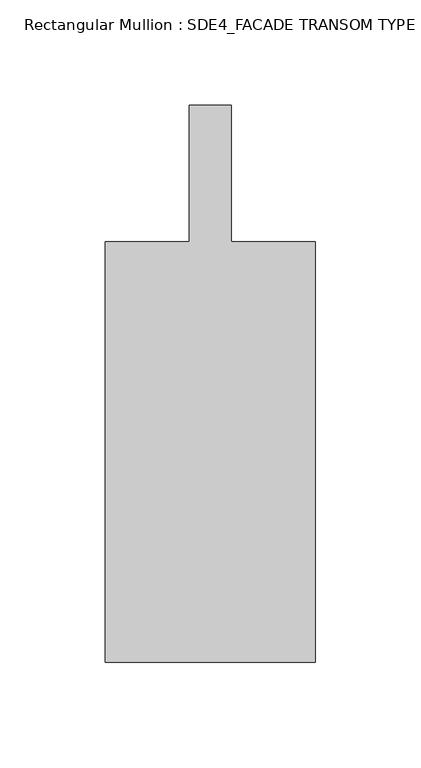
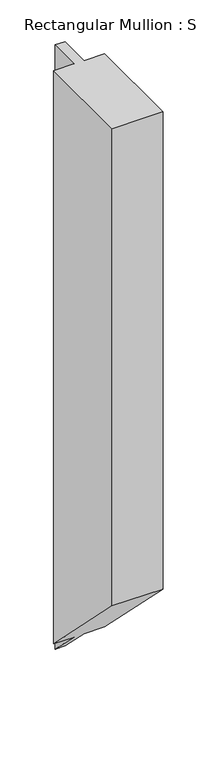
"""IFC4 building model written with IfcOpenShell, lengths in millimetres: member geometry, Rectangular Mullion : SDE4_FACADE TRANSOM TYPE 2."""

from ifc_helpers import new_model, si_unit, origin, place, context, project, spatial, faceted_brep, source, transform, mapped, element, save


def rectangular_mullion_sde4_facade_transom_type_2_1d46e8af(model_context):
    return source(origin(), model_context, "Body", "Brep", [
        faceted_brep([(50.0, -132.5, 0.0), (50.0, 67.5, 0.0), (10.0, 67.5, 0.0), (10.0, 132.5, 0.0), (-10.0, 132.5, 0.0), (-10.0, 67.5, 0.0), (-50.0, 67.5, 0.0), (-50.0, -132.5, 0.0), (50.0, -132.5, -995.0000001), (50.0, 67.5, -1195.0000001), (10.0, 67.5, -1195.0000001), (10.0, 132.5, -1260.0000001), (-10.0, 132.5, -1260.0000001), (-10.0, 67.5, -1195.0000001), (-50.0, 67.5, -1195.0000001), (-50.0, -132.5, -995.0000001)], [[[0, 1, 2, 3, 4, 5, 6, 7]], [[1, 0, 8, 9]], [[2, 1, 9, 10]], [[3, 2, 10, 11]], [[4, 3, 11, 12]], [[5, 4, 12, 13]], [[6, 5, 13, 14]], [[7, 6, 14, 15]], [[0, 7, 15, 8]], [[8, 15, 14, 13, 12, 11, 10, 9]]]),
    ])


if __name__ == "__main__":
    model = new_model("IFC4")
    model_context = context("Model", 3, world=origin())
    ifc_project = project(units=[si_unit("LENGTHUNIT", "METRE", prefix="MILLI")], contexts=[model_context])
    site = spatial("IfcSite", under=ifc_project)
    building = spatial("IfcBuilding", under=site)
    placement = place(None, origin())
    rectangular_mullion_sde4_facade_transom_type_2_shape = rectangular_mullion_sde4_facade_transom_type_2_1d46e8af(model_context)
    element("IfcMember", 1, ObjectType="Rectangular Mullion : SDE4_FACADE TRANSOM TYPE 2", at=placement, inside=building, context=model_context, shape_type="MappedRepresentation", body=[
        mapped(rectangular_mullion_sde4_facade_transom_type_2_shape, transform((0.0, 0.0, 0.0), x_axis=(1.0, 0.0, 0.0), y_axis=(0.0, 1.0, 0.0), z_axis=(0.0, 0.0, 1.0))),
    ])
    save(model, "model.ifc")

# Revit data of these elements
# Type "Rectangular Mullion : SDE4_FACADE TRANSOM TYPE 2"
#   built-in parameter 1007322 = 0.869423 (stored number, unit not read)
#   built-in parameter 1007321 = 0.164042 (stored number, unit not read)
#   built-in parameter 1007320 = 0.164042 (stored number, unit not read)
